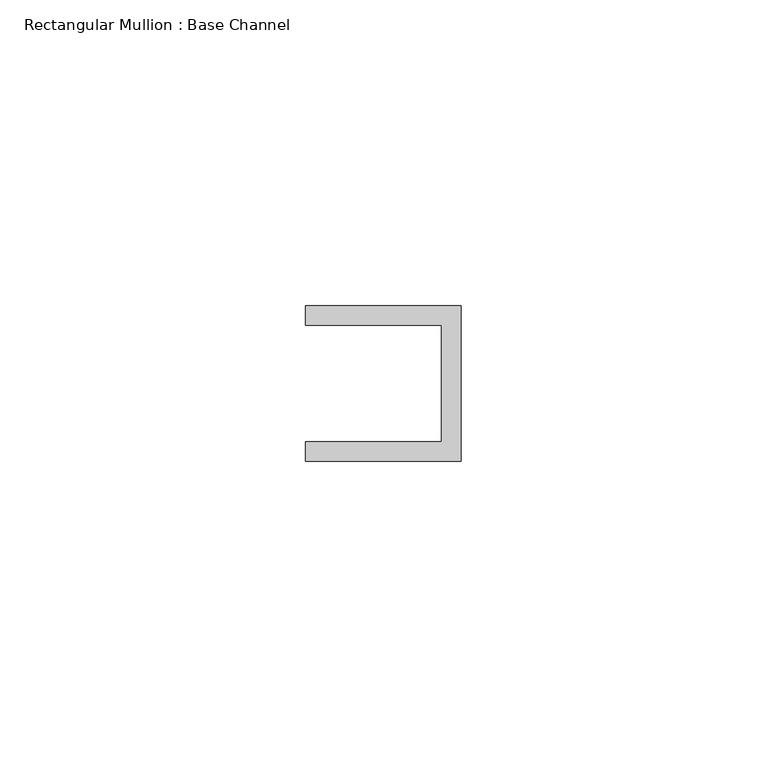
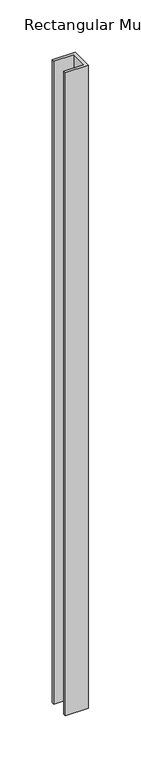
"""IFC4 building model written with IfcOpenShell, lengths in millimetres: member geometry, Rectangular Mullion : Base Channel."""

import ifcopenshell
import ifcopenshell.guid

model = None  # the IFC model being written
_history = None  # IfcOwnerHistory: only IFC2X3 demands one
_inside = {}  # id of a spatial element -> (the spatial element, [elements in it])
_under = {}  # id of a project, library or spatial element -> (it, [spatial elements below it])
_declared = {}  # id of a project -> (the project, [libraries it declares])
_typed = {}  # id of a type object -> (the type object, [elements of that type])
_made_of = {}  # id of a material, layer set ... -> (it, [elements and type objects made of it])


def new_model(schema):
    """Start an empty IFC model of exactly this schema.

    Asked for "IFC4X3", IfcOpenShell would pick the latest addendum, in which some entities
    have other attributes; the version numbers below select the first issue.
    IFC2X3 requires an IfcOwnerHistory on every rooted entity: one is made here for all.
    """
    global model, _history
    if schema == "IFC4X3":
        model = ifcopenshell.file(schema_version=(4, 3, 0, 0))
    else:
        model = ifcopenshell.file(schema=schema)
    _inside.clear()
    _under.clear()
    _declared.clear()
    _typed.clear()
    _made_of.clear()
    _history = None
    if model.schema == "IFC2X3":
        org = make("IfcOrganization", Name="unknown")
        user = make(
            "IfcPersonAndOrganization",
            ThePerson=make("IfcPerson", FamilyName="unknown"),
            TheOrganization=org,
        )
        app = make(
            "IfcApplication",
            ApplicationDeveloper=org,
            Version="unknown",
            ApplicationFullName="unknown",
            ApplicationIdentifier="unknown",
        )
        _history = make(
            "IfcOwnerHistory",
            OwningUser=user,
            OwningApplication=app,
            ChangeAction="ADDED",
            CreationDate=0,
        )
    return model


def make(cls, **values):
    """One entity of the class cls with the attributes given. An attribute that is None is left unset."""
    return model.create_entity(
        cls, **{name: value for name, value in values.items() if value is not None}
    )


def rooted(cls, **values):
    """An entity with a GlobalId (a new one), such as an element, a storey or a relation."""
    return make(cls, GlobalId=ifcopenshell.guid.new(), OwnerHistory=_history, **values)


def si_unit(unit_type, name, prefix=None):
    """IfcSIUnit, for example si_unit("LENGTHUNIT", "METRE", prefix="MILLI")."""
    return make("IfcSIUnit", UnitType=unit_type, Prefix=prefix, Name=name)


def assignment(units):
    """IfcUnitAssignment: the units of a project."""
    return None if units is None else make("IfcUnitAssignment", Units=units)


def point(xyz):
    """IfcCartesianPoint."""
    return None if xyz is None else make("IfcCartesianPoint", Coordinates=xyz)


def direction(xyz):
    """IfcDirection."""
    return None if xyz is None else make("IfcDirection", DirectionRatios=xyz)


def frame(location, z_axis=None, x_axis=None):
    """IfcAxis2Placement3D, a coordinate frame: its origin and axes. An axis left out is left unset."""
    return make(
        "IfcAxis2Placement3D",
        Location=point(location),
        Axis=direction(z_axis),
        RefDirection=direction(x_axis),
    )


def origin():
    """The frame at (0, 0, 0) with its axes left unset."""
    return frame((0.0, 0.0, 0.0))


def place(relative_to, where):
    """IfcLocalPlacement: puts the frame where relative to a parent placement (None: the world)."""
    return make(
        "IfcLocalPlacement", PlacementRelTo=relative_to, RelativePlacement=where
    )


def context(
    kind, dimensions, precision=None, world=None, true_north=None, identifier=None
):
    """IfcGeometricRepresentationContext, for example the 3D "Model" context."""
    return make(
        "IfcGeometricRepresentationContext",
        ContextIdentifier=identifier,
        ContextType=kind,
        CoordinateSpaceDimension=dimensions,
        Precision=precision,
        WorldCoordinateSystem=world,
        TrueNorth=true_north,
    )


def project(units=None, contexts=None):
    """IfcProject with its units and contexts."""
    return rooted(
        "IfcProject",
        Name="project",
        RepresentationContexts=contexts,
        UnitsInContext=assignment(units),
    )


def spatial(cls, under=None, at=None, **own):
    """A site, building, storey or space (cls), placed at a placement, below another one or the project."""
    s = rooted(cls, ObjectPlacement=at, **own)
    if under is not None:
        _under.setdefault(under.id(), (under, []))[1].append(s)
    return s


def polyline(points):
    """IfcPolyline through the points."""
    return make("IfcPolyline", Points=[point(p) for p in points])


def outline(outer, holes=None, kind="AREA"):
    """IfcArbitraryClosedProfileDef: a profile drawn as a closed curve; with holes, ...WithVoids."""
    if holes is None:
        return make("IfcArbitraryClosedProfileDef", ProfileType=kind, OuterCurve=outer)
    return make(
        "IfcArbitraryProfileDefWithVoids",
        ProfileType=kind,
        OuterCurve=outer,
        InnerCurves=holes,
    )


def extrude(swept, where, along, depth):
    """IfcExtrudedAreaSolid: the profile swept, set in the frame where, extruded along a direction by depth."""
    return make(
        "IfcExtrudedAreaSolid",
        SweptArea=swept,
        Position=where,
        ExtrudedDirection=direction(along),
        Depth=depth,
    )


def shape(context_of_items, identifier, shape_type, items):
    """IfcShapeRepresentation: the items that make up one representation, for example the "Body"."""
    return make(
        "IfcShapeRepresentation",
        ContextOfItems=context_of_items,
        RepresentationIdentifier=identifier,
        RepresentationType=shape_type,
        Items=items,
    )


def source(mapping_origin, context_of_items, identifier, shape_type, items):
    """IfcRepresentationMap: a shape defined once, which mapped items show again and again."""
    return make(
        "IfcRepresentationMap",
        MappingOrigin=mapping_origin,
        MappedRepresentation=shape(context_of_items, identifier, shape_type, items),
    )


def transform(
    local_origin,
    x_axis=None,
    y_axis=None,
    z_axis=None,
    scale=None,
    scale2=None,
    scale3=None,
    uniform=True,
):
    """IfcCartesianTransformationOperator3D, or its non-uniform kind. x_axis, y_axis, z_axis: its Axis1, 2, 3."""
    if uniform:
        return make(
            "IfcCartesianTransformationOperator3D",
            Axis1=direction(x_axis),
            Axis2=direction(y_axis),
            LocalOrigin=point(local_origin),
            Scale=scale,
            Axis3=direction(z_axis),
        )
    return make(
        "IfcCartesianTransformationOperator3DnonUniform",
        Axis1=direction(x_axis),
        Axis2=direction(y_axis),
        LocalOrigin=point(local_origin),
        Scale=scale,
        Axis3=direction(z_axis),
        Scale2=scale2,
        Scale3=scale3,
    )


def mapped(mapping_source, mapping_target):
    """IfcMappedItem: shows the shape of a source again, moved by a transform."""
    return make(
        "IfcMappedItem", MappingSource=mapping_source, MappingTarget=mapping_target
    )


def made_of(thing, what):
    """Note that an element or type object is made of a material, layer set ...; save() writes the relation."""
    if what is not None:
        _made_of.setdefault(what.id(), (what, []))[1].append(thing)
    return thing


def element(
    cls,
    number,
    at=None,
    inside=None,
    cuts=None,
    type_object=None,
    material=None,
    context=None,
    identifier="Body",
    shape_type=None,
    held_by="IfcProductDefinitionShape",
    body=None,
    shapes=None,
    **own,
):
    """One element of the class cls, such as IfcWall. Its Tag is "e" and its number.

    at: its placement. inside: the storey or other place that contains it. cuts: it is an
    opening in that element (IfcRelVoidsElement). A single representation is given by context,
    identifier, shape_type and body (its items); several are given by shapes. held_by: the class
    of the entity that holds the representations. save() writes the other relations.
    """
    e = rooted(cls, Tag="e%d" % number, ObjectPlacement=at, **own)
    if body is not None:
        shapes = [shape(context, identifier, shape_type, body)]
    if shapes is not None:
        e.Representation = make(held_by, Representations=shapes)
    if inside is not None:
        _inside.setdefault(inside.id(), (inside, []))[1].append(e)
    if cuts is not None:
        rooted(
            "IfcRelVoidsElement", RelatingBuildingElement=cuts, RelatedOpeningElement=e
        )
    if type_object is not None:
        _typed.setdefault(type_object.id(), (type_object, []))[1].append(e)
    return made_of(e, material)


def aggregate(whole, parts):
    """IfcRelAggregates: a whole, such as a stair, and the parts it consists of."""
    return rooted("IfcRelAggregates", RelatingObject=whole, RelatedObjects=parts)


def save(model, path):
    """Write the relations noted so far, then the file.

    IfcRelAggregates (storeys below a building ...), IfcRelContainedInSpatialStructure (elements
    in a storey), IfcRelDefinesByType, IfcRelAssociatesMaterial and IfcRelDeclares: one each for
    every whole, place, type object, material and project.
    """
    for whole, parts in _under.values():
        aggregate(whole, parts)
    for where, things in _inside.values():
        rooted(
            "IfcRelContainedInSpatialStructure",
            RelatedElements=things,
            RelatingStructure=where,
        )
    for kind, things in _typed.values():
        rooted("IfcRelDefinesByType", RelatedObjects=things, RelatingType=kind)
    for what, things in _made_of.values():
        rooted("IfcRelAssociatesMaterial", RelatedObjects=things, RelatingMaterial=what)
    for by, libraries in _declared.values():
        rooted("IfcRelDeclares", RelatingContext=by, RelatedDefinitions=libraries)
    model.write(path)


def rectangular_mullion_base_channel_f40c63a1(model_context):
    return source(origin(), model_context, "Body", "SweptSolid", [
        extrude(outline(polyline([(0.0, -12.7), (-25.4, -12.7), (-25.4, -9.525), (-3.175, -9.525), (-3.175, 9.525), (-25.4, 9.525), (-25.4, 12.7), (0.0, 12.7), (0.0, -12.7)])), frame((0.0, 0.0, -751.4166667), z_axis=(0.0, 0.0, 1.0), x_axis=(1.0, 0.0, 0.0)), (0.0, 0.0, 1.0), 751.4166667),
    ])


if __name__ == "__main__":
    model = new_model("IFC4")
    model_context = context("Model", 3, world=origin())
    ifc_project = project(units=[si_unit("LENGTHUNIT", "METRE", prefix="MILLI")], contexts=[model_context])
    site = spatial("IfcSite", under=ifc_project)
    building = spatial("IfcBuilding", under=site)
    placement = place(None, origin())
    rectangular_mullion_base_channel_shape = rectangular_mullion_base_channel_f40c63a1(model_context)
    element("IfcMember", 1, ObjectType="Rectangular Mullion : Base Channel", at=placement, inside=building, context=model_context, shape_type="MappedRepresentation", body=[
        mapped(rectangular_mullion_base_channel_shape, transform((0.0, 0.0, 0.0), x_axis=(1.0, 0.0, 0.0), y_axis=(0.0, 1.0, 0.0), z_axis=(0.0, 0.0, 1.0))),
    ])
    save(model, "model.ifc")

# Revit data of these elements
# Type "Rectangular Mullion : Base Channel"
#   built-in parameter 1007322 = 0.0833333 (stored number, unit not read)
#   built-in parameter 1007321 = 0.0416667 (stored number, unit not read)
#   built-in parameter 1007320 = -0.03125 (stored number, unit not read)
# Element 1 (IfcMember, "Rectangular Mullion : Base Channel")
#   Materials on its faces: "ALUM"
# Materials
#   "ALUM": class "Generic", colour RGB 157 157 157, transparency 0, Cost = 0
